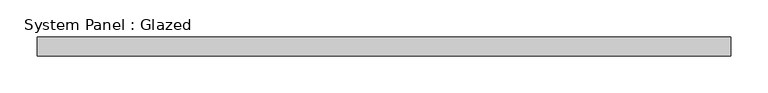
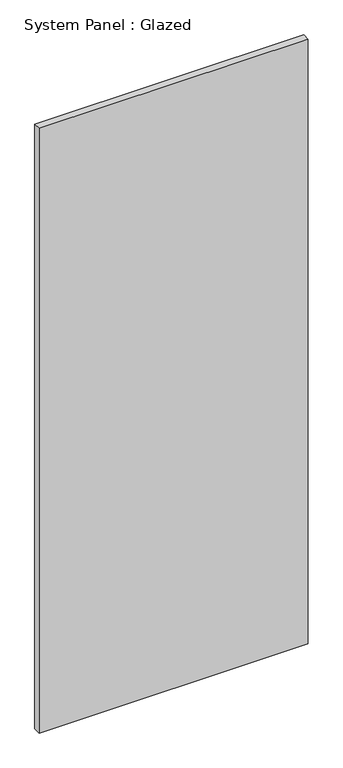
"""IFC4 building model written with IfcOpenShell, lengths in millimetres: plate geometry, System Panel : Glazed."""

from ifc_helpers import new_model, si_unit, origin, origin_with_axes, place, context, project, spatial, polyline, outline, extrude, source, transform, mapped, element, save


def system_panel_glazed_c3e5734e(model_context):
    return source(origin(), model_context, "Body", "SweptSolid", [
        extrude(outline(polyline([(466.7250001, -44.45), (-466.7250001, -44.45), (-466.7250001, -19.05), (466.7250001, -19.05), (466.7250001, -44.45)])), origin_with_axes(), (0.0, 0.0, 1.0), 2216.15),
    ])


if __name__ == "__main__":
    model = new_model("IFC4")
    model_context = context("Model", 3, world=origin())
    ifc_project = project(units=[si_unit("LENGTHUNIT", "METRE", prefix="MILLI")], contexts=[model_context])
    site = spatial("IfcSite", under=ifc_project)
    building = spatial("IfcBuilding", under=site)
    placement = place(None, origin())
    system_panel_glazed_shape = system_panel_glazed_c3e5734e(model_context)
    element("IfcPlate", 1, ObjectType="System Panel : Glazed", at=placement, inside=building, context=model_context, shape_type="MappedRepresentation", body=[
        mapped(system_panel_glazed_shape, transform((0.0, 0.0, 0.0), x_axis=(1.0, 0.0, 0.0), y_axis=(0.0, 1.0, 0.0), z_axis=(0.0, 0.0, 1.0))),
    ])
    save(model, "model.ifc")

# Revit data of these elements
# Type "System Panel : Glazed"
#   Construction Type Id = "GSP4R"
#   Analytic Construction = "1/8 in Pilkington single glazing"
#   Visual Light Transmittance = 0.9
#   Solar Heat Gain Coefficient = 0.86
#   Heat Transfer Coefficient (U) = 1.18115 BTU/(h·ft²·°F)
#   Define Thermal Properties by = 1
# Element 1 (IfcPlate, "System Panel : Glazed")
#   Materials on its faces: "Glass"
# Materials
#   "Glass": class "Glass", colour RGB 0 128 192, transparency 0.75, Description = "Soda Lime Glass", Cost = 0
